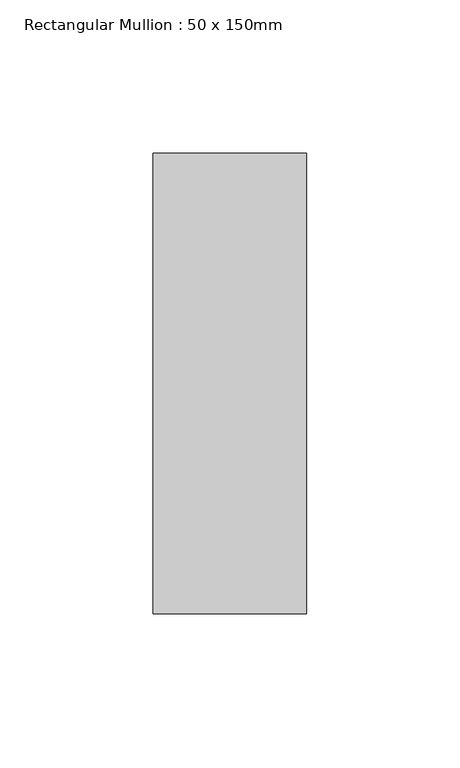
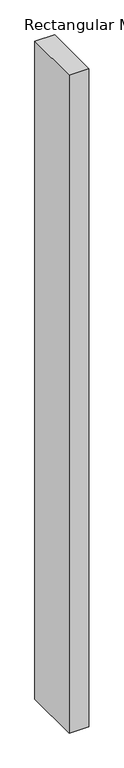
"""IFC4 building model written with IfcOpenShell, lengths in millimetres: member geometry, Rectangular Mullion : 50 x 150mm."""

from ifc_helpers import new_model, si_unit, frame, origin, place, context, project, spatial, polyline, outline, extrude, source, transform, mapped, element, save


def rectangular_mullion_50_x_150mm_267d0d1f(model_context):
    return source(origin(), model_context, "Body", "SweptSolid", [
        extrude(outline(polyline([(25.0, 75.0), (25.0, -75.0), (-25.0, -75.0), (-25.0, 75.0), (25.0, 75.0)])), frame((0.0, 0.0, -1759.0), z_axis=(0.0, 0.0, 1.0), x_axis=(1.0, 0.0, 0.0)), (0.0, 0.0, 1.0), 1759.0),
    ])


if __name__ == "__main__":
    model = new_model("IFC4")
    model_context = context("Model", 3, world=origin())
    ifc_project = project(units=[si_unit("LENGTHUNIT", "METRE", prefix="MILLI")], contexts=[model_context])
    site = spatial("IfcSite", under=ifc_project)
    building = spatial("IfcBuilding", under=site)
    placement = place(None, origin())
    rectangular_mullion_50_x_150mm_shape = rectangular_mullion_50_x_150mm_267d0d1f(model_context)
    element("IfcMember", 1, ObjectType="Rectangular Mullion : 50 x 150mm", at=placement, inside=building, context=model_context, shape_type="MappedRepresentation", body=[
        mapped(rectangular_mullion_50_x_150mm_shape, transform((0.0, 0.0, 0.0), x_axis=(1.0, 0.0, 0.0), y_axis=(0.0, 1.0, 0.0), z_axis=(0.0, 0.0, 1.0))),
    ])
    save(model, "model.ifc")

# Revit data of these elements
# Type "Rectangular Mullion : 50 x 150mm"
#   Keynote = "H11"
#   built-in parameter 1007304 = 0.492126 (stored number, unit not read)
#   built-in parameter 1007301 = 0.082021 (stored number, unit not read)
#   built-in parameter 1007300 = 0.082021 (stored number, unit not read)
# Element 1 (IfcMember, "Rectangular Mullion : 50 x 150mm")
#   Materials on its faces: "Aluminium"
# Materials
#   "Aluminium": class "Metal", colour RGB 247 247 247, transparency 0, Description = "Aluminium 6061", Cost = 0
